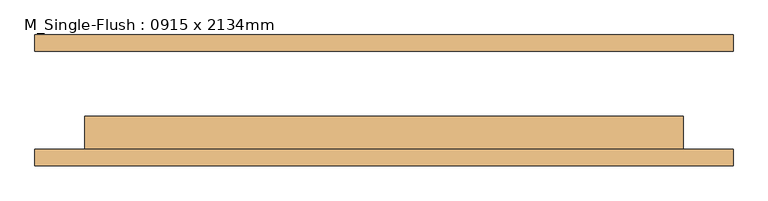
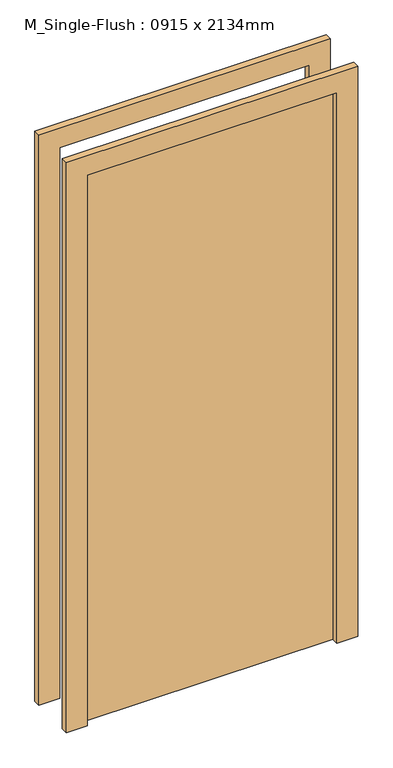
"""IFC4 building model written with IfcOpenShell, lengths in millimetres: door geometry, M_Single-Flush : 0915 x 2134mm."""

import ifcopenshell
import ifcopenshell.guid

model = None  # the IFC model being written
_history = None  # IfcOwnerHistory: only IFC2X3 demands one
_inside = {}  # id of a spatial element -> (the spatial element, [elements in it])
_under = {}  # id of a project, library or spatial element -> (it, [spatial elements below it])
_declared = {}  # id of a project -> (the project, [libraries it declares])
_typed = {}  # id of a type object -> (the type object, [elements of that type])
_made_of = {}  # id of a material, layer set ... -> (it, [elements and type objects made of it])


def new_model(schema):
    """Start an empty IFC model of exactly this schema.

    Asked for "IFC4X3", IfcOpenShell would pick the latest addendum, in which some entities
    have other attributes; the version numbers below select the first issue.
    IFC2X3 requires an IfcOwnerHistory on every rooted entity: one is made here for all.
    """
    global model, _history
    if schema == "IFC4X3":
        model = ifcopenshell.file(schema_version=(4, 3, 0, 0))
    else:
        model = ifcopenshell.file(schema=schema)
    _inside.clear()
    _under.clear()
    _declared.clear()
    _typed.clear()
    _made_of.clear()
    _history = None
    if model.schema == "IFC2X3":
        org = make("IfcOrganization", Name="unknown")
        user = make(
            "IfcPersonAndOrganization",
            ThePerson=make("IfcPerson", FamilyName="unknown"),
            TheOrganization=org,
        )
        app = make(
            "IfcApplication",
            ApplicationDeveloper=org,
            Version="unknown",
            ApplicationFullName="unknown",
            ApplicationIdentifier="unknown",
        )
        _history = make(
            "IfcOwnerHistory",
            OwningUser=user,
            OwningApplication=app,
            ChangeAction="ADDED",
            CreationDate=0,
        )
    return model


def make(cls, **values):
    """One entity of the class cls with the attributes given. An attribute that is None is left unset."""
    return model.create_entity(
        cls, **{name: value for name, value in values.items() if value is not None}
    )


def rooted(cls, **values):
    """An entity with a GlobalId (a new one), such as an element, a storey or a relation."""
    return make(cls, GlobalId=ifcopenshell.guid.new(), OwnerHistory=_history, **values)


def si_unit(unit_type, name, prefix=None):
    """IfcSIUnit, for example si_unit("LENGTHUNIT", "METRE", prefix="MILLI")."""
    return make("IfcSIUnit", UnitType=unit_type, Prefix=prefix, Name=name)


def assignment(units):
    """IfcUnitAssignment: the units of a project."""
    return None if units is None else make("IfcUnitAssignment", Units=units)


def point(xyz):
    """IfcCartesianPoint."""
    return None if xyz is None else make("IfcCartesianPoint", Coordinates=xyz)


def direction(xyz):
    """IfcDirection."""
    return None if xyz is None else make("IfcDirection", DirectionRatios=xyz)


def frame(location, z_axis=None, x_axis=None):
    """IfcAxis2Placement3D, a coordinate frame: its origin and axes. An axis left out is left unset."""
    return make(
        "IfcAxis2Placement3D",
        Location=point(location),
        Axis=direction(z_axis),
        RefDirection=direction(x_axis),
    )


def origin():
    """The frame at (0, 0, 0) with its axes left unset."""
    return frame((0.0, 0.0, 0.0))


def origin_with_axes():
    """The frame at (0, 0, 0) with the z axis (0, 0, 1) and the x axis (1, 0, 0) written out."""
    return frame((0.0, 0.0, 0.0), z_axis=(0.0, 0.0, 1.0), x_axis=(1.0, 0.0, 0.0))


def place(relative_to, where):
    """IfcLocalPlacement: puts the frame where relative to a parent placement (None: the world)."""
    return make(
        "IfcLocalPlacement", PlacementRelTo=relative_to, RelativePlacement=where
    )


def context(
    kind, dimensions, precision=None, world=None, true_north=None, identifier=None
):
    """IfcGeometricRepresentationContext, for example the 3D "Model" context."""
    return make(
        "IfcGeometricRepresentationContext",
        ContextIdentifier=identifier,
        ContextType=kind,
        CoordinateSpaceDimension=dimensions,
        Precision=precision,
        WorldCoordinateSystem=world,
        TrueNorth=true_north,
    )


def project(units=None, contexts=None):
    """IfcProject with its units and contexts."""
    return rooted(
        "IfcProject",
        Name="project",
        RepresentationContexts=contexts,
        UnitsInContext=assignment(units),
    )


def spatial(cls, under=None, at=None, **own):
    """A site, building, storey or space (cls), placed at a placement, below another one or the project."""
    s = rooted(cls, ObjectPlacement=at, **own)
    if under is not None:
        _under.setdefault(under.id(), (under, []))[1].append(s)
    return s


def polyline(points):
    """IfcPolyline through the points."""
    return make("IfcPolyline", Points=[point(p) for p in points])


def outline(outer, holes=None, kind="AREA"):
    """IfcArbitraryClosedProfileDef: a profile drawn as a closed curve; with holes, ...WithVoids."""
    if holes is None:
        return make("IfcArbitraryClosedProfileDef", ProfileType=kind, OuterCurve=outer)
    return make(
        "IfcArbitraryProfileDefWithVoids",
        ProfileType=kind,
        OuterCurve=outer,
        InnerCurves=holes,
    )


def extrude(swept, where, along, depth):
    """IfcExtrudedAreaSolid: the profile swept, set in the frame where, extruded along a direction by depth."""
    return make(
        "IfcExtrudedAreaSolid",
        SweptArea=swept,
        Position=where,
        ExtrudedDirection=direction(along),
        Depth=depth,
    )


def shape(context_of_items, identifier, shape_type, items):
    """IfcShapeRepresentation: the items that make up one representation, for example the "Body"."""
    return make(
        "IfcShapeRepresentation",
        ContextOfItems=context_of_items,
        RepresentationIdentifier=identifier,
        RepresentationType=shape_type,
        Items=items,
    )


def source(mapping_origin, context_of_items, identifier, shape_type, items):
    """IfcRepresentationMap: a shape defined once, which mapped items show again and again."""
    return make(
        "IfcRepresentationMap",
        MappingOrigin=mapping_origin,
        MappedRepresentation=shape(context_of_items, identifier, shape_type, items),
    )


def transform(
    local_origin,
    x_axis=None,
    y_axis=None,
    z_axis=None,
    scale=None,
    scale2=None,
    scale3=None,
    uniform=True,
):
    """IfcCartesianTransformationOperator3D, or its non-uniform kind. x_axis, y_axis, z_axis: its Axis1, 2, 3."""
    if uniform:
        return make(
            "IfcCartesianTransformationOperator3D",
            Axis1=direction(x_axis),
            Axis2=direction(y_axis),
            LocalOrigin=point(local_origin),
            Scale=scale,
            Axis3=direction(z_axis),
        )
    return make(
        "IfcCartesianTransformationOperator3DnonUniform",
        Axis1=direction(x_axis),
        Axis2=direction(y_axis),
        LocalOrigin=point(local_origin),
        Scale=scale,
        Axis3=direction(z_axis),
        Scale2=scale2,
        Scale3=scale3,
    )


def mapped(mapping_source, mapping_target):
    """IfcMappedItem: shows the shape of a source again, moved by a transform."""
    return make(
        "IfcMappedItem", MappingSource=mapping_source, MappingTarget=mapping_target
    )


def made_of(thing, what):
    """Note that an element or type object is made of a material, layer set ...; save() writes the relation."""
    if what is not None:
        _made_of.setdefault(what.id(), (what, []))[1].append(thing)
    return thing


def element(
    cls,
    number,
    at=None,
    inside=None,
    cuts=None,
    type_object=None,
    material=None,
    context=None,
    identifier="Body",
    shape_type=None,
    held_by="IfcProductDefinitionShape",
    body=None,
    shapes=None,
    **own,
):
    """One element of the class cls, such as IfcWall. Its Tag is "e" and its number.

    at: its placement. inside: the storey or other place that contains it. cuts: it is an
    opening in that element (IfcRelVoidsElement). A single representation is given by context,
    identifier, shape_type and body (its items); several are given by shapes. held_by: the class
    of the entity that holds the representations. save() writes the other relations.
    """
    e = rooted(cls, Tag="e%d" % number, ObjectPlacement=at, **own)
    if body is not None:
        shapes = [shape(context, identifier, shape_type, body)]
    if shapes is not None:
        e.Representation = make(held_by, Representations=shapes)
    if inside is not None:
        _inside.setdefault(inside.id(), (inside, []))[1].append(e)
    if cuts is not None:
        rooted(
            "IfcRelVoidsElement", RelatingBuildingElement=cuts, RelatedOpeningElement=e
        )
    if type_object is not None:
        _typed.setdefault(type_object.id(), (type_object, []))[1].append(e)
    return made_of(e, material)


def aggregate(whole, parts):
    """IfcRelAggregates: a whole, such as a stair, and the parts it consists of."""
    return rooted("IfcRelAggregates", RelatingObject=whole, RelatedObjects=parts)


def save(model, path):
    """Write the relations noted so far, then the file.

    IfcRelAggregates (storeys below a building ...), IfcRelContainedInSpatialStructure (elements
    in a storey), IfcRelDefinesByType, IfcRelAssociatesMaterial and IfcRelDeclares: one each for
    every whole, place, type object, material and project.
    """
    for whole, parts in _under.values():
        aggregate(whole, parts)
    for where, things in _inside.values():
        rooted(
            "IfcRelContainedInSpatialStructure",
            RelatedElements=things,
            RelatingStructure=where,
        )
    for kind, things in _typed.values():
        rooted("IfcRelDefinesByType", RelatedObjects=things, RelatingType=kind)
    for what, things in _made_of.values():
        rooted("IfcRelAssociatesMaterial", RelatedObjects=things, RelatingMaterial=what)
    for by, libraries in _declared.values():
        rooted("IfcRelDeclares", RelatingContext=by, RelatedDefinitions=libraries)
    model.write(path)


def m_single_flush_0915_x_2134mm_f3d7f739(model_context):
    return source(origin(), model_context, "Body", "SweptSolid", [
        extrude(outline(polyline([(2210.0, -533.5), (0.0, -533.5), (0.0, -457.5), (2134.0, -457.5), (2134.0, 457.5), (0.0, 457.5), (0.0, 533.5), (2210.0, 533.5), (2210.0, -533.5)])), frame((0.0, -100.0, 0.0), z_axis=(0.0, 1.0, 0.0), x_axis=(0.0, 0.0, 1.0)), (0.0, 0.0, 1.0), 25.0),
        extrude(outline(polyline([(2210.0, 533.5), (2210.0, -533.5), (0.0, -533.5), (0.0, -457.5), (2134.0, -457.5), (2134.0, 457.5), (0.0, 457.5), (0.0, 533.5), (2210.0, 533.5)])), frame((0.0, 75.0, 0.0), z_axis=(0.0, 1.0, 0.0), x_axis=(0.0, 0.0, 1.0)), (0.0, 0.0, 1.0), 25.0),
        extrude(outline(polyline([(457.5, -24.0), (457.5, -75.0), (-457.5, -75.0), (-457.5, -24.0), (457.5, -24.0)])), origin_with_axes(), (0.0, 0.0, 1.0), 2134.0),
    ])


if __name__ == "__main__":
    model = new_model("IFC4")
    model_context = context("Model", 3, world=origin())
    ifc_project = project(units=[si_unit("LENGTHUNIT", "METRE", prefix="MILLI")], contexts=[model_context])
    site = spatial("IfcSite", under=ifc_project)
    building = spatial("IfcBuilding", under=site)
    placement = place(None, origin())
    m_single_flush_0915_x_2134mm_shape = m_single_flush_0915_x_2134mm_f3d7f739(model_context)
    element("IfcDoor", 1, ObjectType="M_Single-Flush : 0915 x 2134mm", at=placement, inside=building, context=model_context, shape_type="MappedRepresentation", body=[
        mapped(m_single_flush_0915_x_2134mm_shape, transform((0.0, 0.0, 0.0), x_axis=(1.0, 0.0, 0.0), y_axis=(0.0, 1.0, 0.0), z_axis=(0.0, 0.0, 1.0))),
    ])
    save(model, "model.ifc")

# Revit data of these elements
# Type "M_Single-Flush : 0915 x 2134mm"
#   Type Mark = "15"
#   Thickness = 0.051 m
#   Height = 2.134 m
#   Trim Projection Ext = 0.025 m
#   Trim Projection Int = 0.025 m
#   Trim Width = 0.076 m
#   Width = 0.915 m
#   Door Material = Door - Panel
#   Frame Material = Door - Frame
#   Function = (empty or 0)
#   Wall Closure = (empty or 0)
# Element 1 (IfcDoor, "M_Single-Flush : 0915 x 2134mm")
#   Materials on its faces: "Door - Frame", "Door - Panel"
# Materials
#   "Door - Panel": class "Wood", colour RGB 114 82 51, transparency 0
#   "Door - Frame": class "Miscellaneous", colour RGB 255 0 128, transparency 0, Cost = 0
